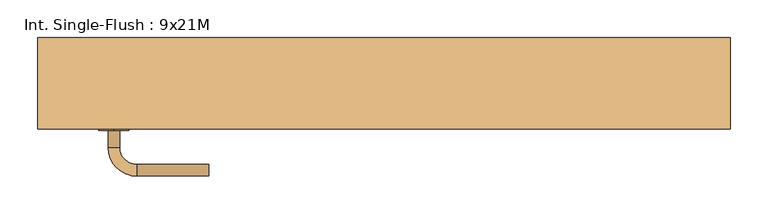
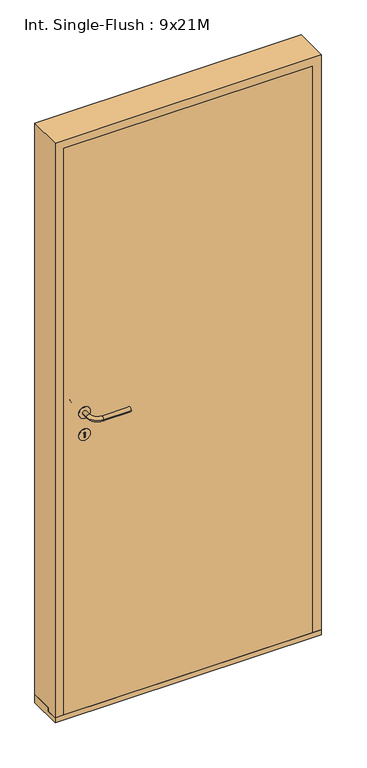
"""IFC4 building model written with IfcOpenShell, lengths in millimetres: door geometry, Int. Single-Flush : 9x21M."""

from ifc_helpers import new_model, si_unit, point, frame, frame_2d, origin, place, context, project, spatial, polyline, circle_curve, ellipse_curve, trimmed, segment, composite_curve, outline, extrude, faceted_brep, source, transform, mapped, element, save
from ifc_brep_helpers import plane_surface, cylinder_surface, revolved_surface, advanced_brep


def int_single_flush_9x21m_9bb4a9f8(model_context):
    return source(origin(), model_context, "Body", "SolidModel", [
        extrude(outline(composite_curve([segment(trimmed(circle_curve(frame_2d((1090.0, -356.0)), 20.0), [point((1070.0, -356.0))], [point((1110.0, -356.0))], False, "CARTESIAN"), True, "CONTINUOUS"), segment(trimmed(circle_curve(frame_2d((1090.0, -356.0)), 20.0), [point((1110.0, -356.0))], [point((1070.0, -356.0))], False, "CARTESIAN"), True, "CONTINUOUS")], self_intersect=False)), frame((0.0, -62.0, 0.0), z_axis=(0.0, 1.0, 0.0), x_axis=(0.0, 0.0, 1.0)), (0.0, 0.0, 1.0), 2.0),
        advanced_brep(
        [(-363.5, -62.0, 1090.0), (-348.5, -62.0, 1090.0), (-348.5, -84.5, 1090.0), (-363.5, -84.5, 1090.0), (-326.0, -107.0, 1090.0), (-326.0, -122.0, 1090.0), (-231.0, -107.0, 1090.0), (-231.0, -122.0, 1090.0)],
        [
            (0, 1, circle_curve(frame((-356.0, -62.0, 1090.0), z_axis=(0.0, 1.0, 0.0), x_axis=(1.0, 0.0, 0.0)), 7.5)),
            (1, 0, circle_curve(frame((-356.0, -62.0, 1090.0), z_axis=(0.0, 1.0, 0.0), x_axis=(1.0, 0.0, 0.0)), 7.5)),
            (1, 2),
            (2, 3, circle_curve(frame((-356.0, -84.5, 1090.0), z_axis=(0.0, 1.0, 0.0), x_axis=(1.0, 0.0, 0.0)), 7.5)),
            (3, 0),
            (3, 2, circle_curve(frame((-356.0, -84.5, 1090.0), z_axis=(0.0, 1.0, 0.0), x_axis=(1.0, 0.0, 0.0)), 7.5)),
            (4, 5, circle_curve(frame((-326.0, -114.5, 1090.0), z_axis=(-1.0, 0.0, 0.0), x_axis=(0.0, 1.0, 0.0)), 7.5)),
            (5, 3, circle_curve(frame((-326.0, -84.5, 1090.0), z_axis=(0.0, 0.0, -1.0), x_axis=(-1.0, 0.0, 0.0)), 37.5)),
            (2, 4, circle_curve(frame((-326.0, -84.5, 1090.0), z_axis=(0.0, 0.0, 1.0), x_axis=(-1.0, 0.0, 0.0)), 22.5)),
            (5, 4, circle_curve(frame((-326.0, -114.5, 1090.0), z_axis=(-1.0, 0.0, 0.0), x_axis=(0.0, 1.0, 0.0)), 7.5)),
            (4, 6),
            (6, 7, circle_curve(frame((-231.0, -114.5, 1090.0), z_axis=(-1.0, 0.0, 0.0), x_axis=(0.0, 1.0, 0.0)), 7.5)),
            (7, 5),
            (7, 6, circle_curve(frame((-231.0, -114.5, 1090.0), z_axis=(-1.0, 0.0, 0.0), x_axis=(0.0, 1.0, 0.0)), 7.5)),
        ],
        [
            plane_surface(frame((-356.0, -62.0, 1090.0), z_axis=(0.0, 1.0, 0.0), x_axis=(0.0, 0.0, -1.0))),
            cylinder_surface(frame((-356.0, -62.0, 1090.0), z_axis=(0.0, 1.0, 0.0), x_axis=(1.0, 0.0, 0.0)), 7.5),
            revolved_surface(trimmed(ellipse_curve(frame((-356.0, -84.5, 1090.0), z_axis=(0.0, -1.0, 0.0), x_axis=(1.0, 0.0, 0.0)), 7.5, 7.5), [point((-363.5, -84.5, 1090.0))], [point((-348.5, -84.5, 1090.0))], True, "CARTESIAN"), (-326.0, -84.5, 1090.0), (0.0, 0.0, -1.0)),
            revolved_surface(trimmed(ellipse_curve(frame((-356.0, -84.5, 1090.0), z_axis=(0.0, -1.0, 0.0), x_axis=(1.0, 0.0, 0.0)), 7.5, 7.5), [point((-348.5, -84.5, 1090.0))], [point((-363.5, -84.5, 1090.0))], True, "CARTESIAN"), (-326.0, -84.5, 1090.0), (0.0, 0.0, -1.0)),
            cylinder_surface(frame((-326.0, -114.5, 1090.0), z_axis=(-1.0, 0.0, 0.0), x_axis=(0.0, 1.0, 0.0)), 7.5),
            plane_surface(frame((-231.0, -114.5, 1090.0), z_axis=(1.0, 0.0, 0.0), x_axis=(0.0, 0.0, -1.0))),
        ],
        [
            (0, [[1, 2]]),
            (1, [[3, 4, 5, -2]]),
            (1, [[-5, 6, -3, -1]]),
            (2, [[7, 8, -4, 9]]),
            (3, [[10, -9, -6, -8]]),
            (4, [[11, 12, 13, -7]]),
            (4, [[-13, 14, -11, -10]]),
            (5, [[-12, -14]]),
        ],
    ),
        extrude(outline(composite_curve([segment(trimmed(circle_curve(frame_2d((1010.0, -356.0)), 20.0), [point((990.0, -356.0))], [point((1030.0, -356.0))], False, "CARTESIAN"), True, "CONTINUOUS"), segment(trimmed(circle_curve(frame_2d((1010.0, -356.0)), 20.0), [point((1030.0, -356.0))], [point((990.0, -356.0))], False, "CARTESIAN"), True, "CONTINUOUS")], self_intersect=False), holes=[composite_curve([segment(trimmed(circle_curve(frame_2d((1015.0, -356.0)), 3.0), [point((1012.4019238, -357.5))], [point((1012.4019238, -354.5))], True, "CARTESIAN"), True, "CONTINUOUS"), segment(polyline([(1012.4019238, -354.5), (1000.0, -354.5), (1000.0, -357.5), (1012.4019238, -357.5)]), True, "CONTINUOUS")], self_intersect=False)]), frame((0.0, -62.0, 0.0), z_axis=(0.0, 1.0, 0.0), x_axis=(0.0, 0.0, 1.0)), (0.0, 0.0, 1.0), 2.0),
        extrude(outline(composite_curve([segment(trimmed(circle_curve(frame_2d((1090.0, -356.0)), 20.0), [point((1070.0, -356.0))], [point((1110.0, -356.0))], False, "CARTESIAN"), True, "CONTINUOUS"), segment(trimmed(circle_curve(frame_2d((1090.0, -356.0)), 20.0), [point((1110.0, -356.0))], [point((1070.0, -356.0))], False, "CARTESIAN"), True, "CONTINUOUS")], self_intersect=False)), frame((0.0, -20.0, 0.0), z_axis=(0.0, 1.0, 0.0), x_axis=(0.0, 0.0, 1.0)), (0.0, 0.0, 1.0), 2.0),
        advanced_brep(
        [(-363.5, -18.0, 1090.0), (-348.5, -18.0, 1090.0), (-363.5, 4.5, 1090.0), (-348.5, 4.5, 1090.0), (-326.0, 27.0, 1090.0), (-326.0, 42.0, 1090.0), (-231.0, 42.0, 1090.0), (-231.0, 27.0, 1090.0)],
        [
            (0, 1, circle_curve(frame((-356.0, -18.0, 1090.0), z_axis=(0.0, -1.0, 0.0), x_axis=(1.0, 0.0, 0.0)), 7.5)),
            (1, 0, circle_curve(frame((-356.0, -18.0, 1090.0), z_axis=(0.0, -1.0, 0.0), x_axis=(1.0, 0.0, 0.0)), 7.5)),
            (0, 2),
            (2, 3, circle_curve(frame((-356.0, 4.5, 1090.0), z_axis=(0.0, -1.0, 0.0), x_axis=(1.0, 0.0, 0.0)), 7.5)),
            (3, 1),
            (3, 2, circle_curve(frame((-356.0, 4.5, 1090.0), z_axis=(0.0, -1.0, 0.0), x_axis=(1.0, 0.0, 0.0)), 7.5)),
            (4, 3, circle_curve(frame((-326.0, 4.5, 1090.0), z_axis=(0.0, 0.0, 1.0), x_axis=(-1.0, 0.0, 0.0)), 22.5)),
            (2, 5, circle_curve(frame((-326.0, 4.5, 1090.0), z_axis=(0.0, 0.0, -1.0), x_axis=(-1.0, 0.0, 0.0)), 37.5)),
            (5, 4, circle_curve(frame((-326.0, 34.5, 1090.0), z_axis=(-1.0, 0.0, 0.0), x_axis=(0.0, -1.0, 0.0)), 7.5)),
            (4, 5, circle_curve(frame((-326.0, 34.5, 1090.0), z_axis=(-1.0, 0.0, 0.0), x_axis=(0.0, -1.0, 0.0)), 7.5)),
            (5, 6),
            (6, 7, circle_curve(frame((-231.0, 34.5, 1090.0), z_axis=(-1.0, 0.0, 0.0), x_axis=(0.0, -1.0, 0.0)), 7.5)),
            (7, 4),
            (7, 6, circle_curve(frame((-231.0, 34.5, 1090.0), z_axis=(-1.0, 0.0, 0.0), x_axis=(0.0, -1.0, 0.0)), 7.5)),
        ],
        [
            plane_surface(frame((-356.0, -18.0, 1090.0), z_axis=(0.0, -1.0, 0.0), x_axis=(0.0, 0.0, -1.0))),
            cylinder_surface(frame((-356.0, -18.0, 1090.0), z_axis=(0.0, -1.0, 0.0), x_axis=(1.0, 0.0, 0.0)), 7.5),
            revolved_surface(trimmed(ellipse_curve(frame((-356.0, 4.5, 1090.0), z_axis=(0.0, -1.0, 0.0), x_axis=(1.0, 0.0, 0.0)), 7.5, 7.5), [point((-363.5, 4.5, 1090.0))], [point((-348.5, 4.5, 1090.0))], True, "CARTESIAN"), (-326.0, 4.5, 1090.0), (0.0, 0.0, -1.0)),
            revolved_surface(trimmed(ellipse_curve(frame((-356.0, 4.5, 1090.0), z_axis=(0.0, -1.0, 0.0), x_axis=(1.0, 0.0, 0.0)), 7.5, 7.5), [point((-348.5, 4.5, 1090.0))], [point((-363.5, 4.5, 1090.0))], True, "CARTESIAN"), (-326.0, 4.5, 1090.0), (0.0, 0.0, -1.0)),
            cylinder_surface(frame((-326.0, 34.5, 1090.0), z_axis=(-1.0, 0.0, 0.0), x_axis=(0.0, -1.0, 0.0)), 7.5),
            plane_surface(frame((-231.0, 34.5, 1090.0), z_axis=(1.0, 0.0, 0.0), x_axis=(0.0, 0.0, -1.0))),
        ],
        [
            (0, [[1, 2]]),
            (1, [[-1, 3, 4, 5]]),
            (1, [[-2, -5, 6, -3]]),
            (2, [[7, -4, 8, 9]]),
            (3, [[-8, -6, -7, 10]]),
            (4, [[-9, 11, 12, 13]]),
            (4, [[-10, -13, 14, -11]]),
            (5, [[-14, -12]]),
        ],
    ),
        extrude(outline(composite_curve([segment(trimmed(circle_curve(frame_2d((1010.0, -356.0)), 20.0), [point((990.0, -356.0))], [point((1030.0, -356.0))], False, "CARTESIAN"), True, "CONTINUOUS"), segment(trimmed(circle_curve(frame_2d((1010.0, -356.0)), 20.0), [point((1030.0, -356.0))], [point((990.0, -356.0))], False, "CARTESIAN"), True, "CONTINUOUS")], self_intersect=False), holes=[composite_curve([segment(trimmed(circle_curve(frame_2d((1015.0, -356.0)), 3.0), [point((1012.4019238, -357.5))], [point((1012.4019238, -354.5))], True, "CARTESIAN"), True, "CONTINUOUS"), segment(polyline([(1012.4019238, -354.5), (1000.0, -354.5), (1000.0, -357.5), (1012.4019238, -357.5)]), True, "CONTINUOUS")], self_intersect=False)]), frame((0.0, -20.0, 0.0), z_axis=(0.0, 1.0, 0.0), x_axis=(0.0, 0.0, 1.0)), (0.0, 0.0, 1.0), 2.0),
        extrude(outline(polyline([(426.0, -20.0), (426.0, -60.0), (-426.0, -60.0), (-426.0, -20.0), (426.0, -20.0)])), frame((0.0, 0.0, 18.0), z_axis=(0.0, 0.0, 1.0), x_axis=(1.0, 0.0, 0.0)), (0.0, 0.0, 1.0), 2052.0),
        faceted_brep([(-426.0, -20.0, 2070.0), (-426.0, -20.0, 30.0), (-414.0, -20.0, 30.0), (-414.0, -20.0, 2058.0), (414.0, -20.0, 2058.0), (414.0, -20.0, 30.0), (426.0, -20.0, 30.0), (426.0, -20.0, 2070.0), (-426.0, -60.0, 2070.0), (-426.0, -60.0, 18.0), (-426.0, -20.0, 18.0), (-456.0, -20.0, 18.0), (-456.0, -20.0, 30.0), (456.0, -20.0, 30.0), (456.0, -20.0, 18.0), (426.0, -20.0, 18.0), (-456.0, -60.0, 18.0), (456.0, -60.0, 18.0), (426.0, -60.0, 18.0), (-456.0, -60.0, 2100.0), (426.0, -60.0, 2070.0), (456.0, -60.0, 2100.0), (414.0, 60.0, 30.0), (456.0, 60.0, 30.0), (-456.0, 60.0, 30.0), (-414.0, 60.0, 30.0), (414.0, 60.0, 2058.0), (-414.0, 60.0, 2058.0), (-456.0, 60.0, 2100.0), (456.0, 60.0, 2100.0)], [[[0, 1, 2, 3, 4, 5, 6, 7]], [[8, 9, 10, 1, 0]], [[1, 10, 11, 12]], [[13, 14, 15, 6]], [[10, 9, 16, 11]], [[14, 17, 18, 15]], [[19, 16, 9, 8, 20, 18, 17, 21]], [[7, 6, 15, 18, 20]], [[6, 5, 22, 23, 13]], [[12, 24, 25, 2, 1]], [[26, 22, 5, 4]], [[3, 2, 25, 27]], [[27, 25, 24, 28, 29, 23, 22, 26]], [[21, 17, 14, 13, 23, 29]], [[28, 24, 12, 11, 16, 19]], [[0, 7, 20, 8]], [[3, 27, 26, 4]], [[28, 19, 21, 29]]]),
        extrude(outline(polyline([(-20.0, 30.0), (60.0, 30.0), (60.0, 0.0), (-60.0, 0.0), (-60.0, 18.0), (-20.0, 18.0), (-20.0, 30.0)])), frame((-456.0, 0.0, 0.0), z_axis=(1.0, 0.0, 0.0), x_axis=(0.0, 1.0, 0.0)), (0.0, 0.0, 1.0), 912.0),
    ])


if __name__ == "__main__":
    model = new_model("IFC4")
    model_context = context("Model", 3, world=origin())
    ifc_project = project(units=[si_unit("LENGTHUNIT", "METRE", prefix="MILLI")], contexts=[model_context])
    site = spatial("IfcSite", under=ifc_project)
    building = spatial("IfcBuilding", under=site)
    placement = place(None, origin())
    int_single_flush_9x21m_shape = int_single_flush_9x21m_9bb4a9f8(model_context)
    element("IfcDoor", 1, ObjectType="Int. Single-Flush : 9x21M", at=placement, inside=building, context=model_context, shape_type="MappedRepresentation", body=[
        mapped(int_single_flush_9x21m_shape, transform((0.0, 0.0, 0.0), x_axis=(1.0, 0.0, 0.0), y_axis=(0.0, 1.0, 0.0), z_axis=(0.0, 0.0, 1.0))),
    ])
    save(model, "model.ifc")

# Revit data of these elements
# Type "Int. Single-Flush : 9x21M"
#   Type Mark = "53"
#   Sound Rating = ""
#   Hinge Side [instance default] = ""
#   Creator Build [instance default] = "2017.0301.0"
#   Creator Organization [instance default] = "© Danish Educational Content"
#   Creator Name [instance default] = "© Erik Falck Jørgensen"
#   Analytic Construction = "<None>"
#   length#3 = 18 mm
#   length#2 = 42 mm
#   length#1 = 0 mm
#   length#4 = 912 mm
#   Thickness = 40 mm
#   Seal Width = 12 mm
#   Rough Width = 912 mm
#   Rough Height = 2100 mm
#   Rabbet Width = 12 mm
#   Rabbet Depth = 40 mm
#   Interior Distance [instance default] = 0 mm
#   Height = 2088 mm
#   Width = 888 mm
#   Handle From Side = 100 mm
#   Handle From Bottom = 1090 mm
#   Exterior Direction [instance default] = 0.00°
#   Case Depth [instance default] = 200 mm
#   Case Width = 30 mm
#   Exterior Distance [instance default] = 0 mm
#   Threshold = yes
#   Sealing = no
#   Hinging = yes
#   Wall Closure = 1
#   Door Panel = no
#   Panel = none
#   Handle Finish = none
#   Handle = element 510752
#   Case/Transom = none
#   Function = (empty or 0)
#   Assembly Code = ""
# Element 1 (IfcDoor, "Int. Single-Flush : 9x21M")
#   Case Depth = 120 mm
#   Materials on its faces: "Stainless Steel, Polished", "Default Frame/Mullion (Interior/Exterior)", "Default Door Panel (Exterior/Interior)"
# Materials
#   "Stainless Steel, Polished": class "Metal", colour RGB 180 180 180, transparency 0, Description = "Rustfri stål, poleret", Cost = 0
#   "Default Frame/Mullion (Interior/Exterior)": class "Generic", colour RGB 205 205 205, transparency 0, Description = "Udefineret karm/ramme materiale", Cost = 0
#   "Default Door Panel (Exterior/Interior)": class "Generic", colour RGB 205 205 205, transparency 0, Description = "Udefineret dørplade materiale", Cost = 0
